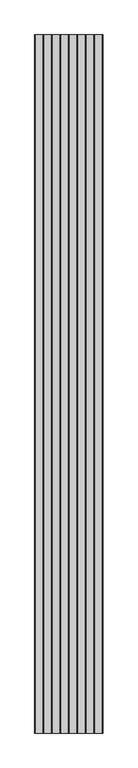
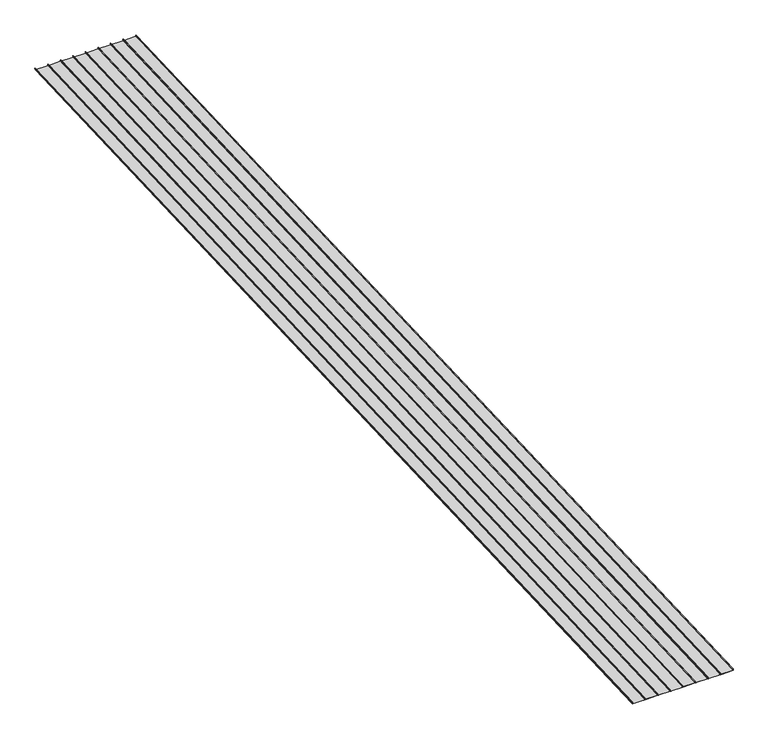
"""IFC4 building model written with IfcOpenShell, lengths in millimetres: proxy geometry, Generic Models 2:Generic Models 2:310765:Generic Models 2:310765 : Generic Models 2:Generic Models 2:310765:8 : Generic Models 2:Generic Models 2:310765:Generic Models 2:310765 : Generic Models 2:Generic Models 2:310765:300385."""

import ifcopenshell
import ifcopenshell.guid

model = None  # the IFC model being written
_history = None  # IfcOwnerHistory: only IFC2X3 demands one
_inside = {}  # id of a spatial element -> (the spatial element, [elements in it])
_under = {}  # id of a project, library or spatial element -> (it, [spatial elements below it])
_declared = {}  # id of a project -> (the project, [libraries it declares])
_typed = {}  # id of a type object -> (the type object, [elements of that type])
_made_of = {}  # id of a material, layer set ... -> (it, [elements and type objects made of it])


def new_model(schema):
    """Start an empty IFC model of exactly this schema.

    Asked for "IFC4X3", IfcOpenShell would pick the latest addendum, in which some entities
    have other attributes; the version numbers below select the first issue.
    IFC2X3 requires an IfcOwnerHistory on every rooted entity: one is made here for all.
    """
    global model, _history
    if schema == "IFC4X3":
        model = ifcopenshell.file(schema_version=(4, 3, 0, 0))
    else:
        model = ifcopenshell.file(schema=schema)
    _inside.clear()
    _under.clear()
    _declared.clear()
    _typed.clear()
    _made_of.clear()
    _history = None
    if model.schema == "IFC2X3":
        org = make("IfcOrganization", Name="unknown")
        user = make(
            "IfcPersonAndOrganization",
            ThePerson=make("IfcPerson", FamilyName="unknown"),
            TheOrganization=org,
        )
        app = make(
            "IfcApplication",
            ApplicationDeveloper=org,
            Version="unknown",
            ApplicationFullName="unknown",
            ApplicationIdentifier="unknown",
        )
        _history = make(
            "IfcOwnerHistory",
            OwningUser=user,
            OwningApplication=app,
            ChangeAction="ADDED",
            CreationDate=0,
        )
    return model


def make(cls, **values):
    """One entity of the class cls with the attributes given. An attribute that is None is left unset."""
    return model.create_entity(
        cls, **{name: value for name, value in values.items() if value is not None}
    )


def rooted(cls, **values):
    """An entity with a GlobalId (a new one), such as an element, a storey or a relation."""
    return make(cls, GlobalId=ifcopenshell.guid.new(), OwnerHistory=_history, **values)


def si_unit(unit_type, name, prefix=None):
    """IfcSIUnit, for example si_unit("LENGTHUNIT", "METRE", prefix="MILLI")."""
    return make("IfcSIUnit", UnitType=unit_type, Prefix=prefix, Name=name)


def assignment(units):
    """IfcUnitAssignment: the units of a project."""
    return None if units is None else make("IfcUnitAssignment", Units=units)


def point(xyz):
    """IfcCartesianPoint."""
    return None if xyz is None else make("IfcCartesianPoint", Coordinates=xyz)


def direction(xyz):
    """IfcDirection."""
    return None if xyz is None else make("IfcDirection", DirectionRatios=xyz)


def frame(location, z_axis=None, x_axis=None):
    """IfcAxis2Placement3D, a coordinate frame: its origin and axes. An axis left out is left unset."""
    return make(
        "IfcAxis2Placement3D",
        Location=point(location),
        Axis=direction(z_axis),
        RefDirection=direction(x_axis),
    )


def origin():
    """The frame at (0, 0, 0) with its axes left unset."""
    return frame((0.0, 0.0, 0.0))


def place(relative_to, where):
    """IfcLocalPlacement: puts the frame where relative to a parent placement (None: the world)."""
    return make(
        "IfcLocalPlacement", PlacementRelTo=relative_to, RelativePlacement=where
    )


def context(
    kind, dimensions, precision=None, world=None, true_north=None, identifier=None
):
    """IfcGeometricRepresentationContext, for example the 3D "Model" context."""
    return make(
        "IfcGeometricRepresentationContext",
        ContextIdentifier=identifier,
        ContextType=kind,
        CoordinateSpaceDimension=dimensions,
        Precision=precision,
        WorldCoordinateSystem=world,
        TrueNorth=true_north,
    )


def project(units=None, contexts=None):
    """IfcProject with its units and contexts."""
    return rooted(
        "IfcProject",
        Name="project",
        RepresentationContexts=contexts,
        UnitsInContext=assignment(units),
    )


def spatial(cls, under=None, at=None, **own):
    """A site, building, storey or space (cls), placed at a placement, below another one or the project."""
    s = rooted(cls, ObjectPlacement=at, **own)
    if under is not None:
        _under.setdefault(under.id(), (under, []))[1].append(s)
    return s


def polyline(points):
    """IfcPolyline through the points."""
    return make("IfcPolyline", Points=[point(p) for p in points])


def outline(outer, holes=None, kind="AREA"):
    """IfcArbitraryClosedProfileDef: a profile drawn as a closed curve; with holes, ...WithVoids."""
    if holes is None:
        return make("IfcArbitraryClosedProfileDef", ProfileType=kind, OuterCurve=outer)
    return make(
        "IfcArbitraryProfileDefWithVoids",
        ProfileType=kind,
        OuterCurve=outer,
        InnerCurves=holes,
    )


def extrude(swept, where, along, depth):
    """IfcExtrudedAreaSolid: the profile swept, set in the frame where, extruded along a direction by depth."""
    return make(
        "IfcExtrudedAreaSolid",
        SweptArea=swept,
        Position=where,
        ExtrudedDirection=direction(along),
        Depth=depth,
    )


def shape(context_of_items, identifier, shape_type, items):
    """IfcShapeRepresentation: the items that make up one representation, for example the "Body"."""
    return make(
        "IfcShapeRepresentation",
        ContextOfItems=context_of_items,
        RepresentationIdentifier=identifier,
        RepresentationType=shape_type,
        Items=items,
    )


def source(mapping_origin, context_of_items, identifier, shape_type, items):
    """IfcRepresentationMap: a shape defined once, which mapped items show again and again."""
    return make(
        "IfcRepresentationMap",
        MappingOrigin=mapping_origin,
        MappedRepresentation=shape(context_of_items, identifier, shape_type, items),
    )


def transform(
    local_origin,
    x_axis=None,
    y_axis=None,
    z_axis=None,
    scale=None,
    scale2=None,
    scale3=None,
    uniform=True,
):
    """IfcCartesianTransformationOperator3D, or its non-uniform kind. x_axis, y_axis, z_axis: its Axis1, 2, 3."""
    if uniform:
        return make(
            "IfcCartesianTransformationOperator3D",
            Axis1=direction(x_axis),
            Axis2=direction(y_axis),
            LocalOrigin=point(local_origin),
            Scale=scale,
            Axis3=direction(z_axis),
        )
    return make(
        "IfcCartesianTransformationOperator3DnonUniform",
        Axis1=direction(x_axis),
        Axis2=direction(y_axis),
        LocalOrigin=point(local_origin),
        Scale=scale,
        Axis3=direction(z_axis),
        Scale2=scale2,
        Scale3=scale3,
    )


def mapped(mapping_source, mapping_target):
    """IfcMappedItem: shows the shape of a source again, moved by a transform."""
    return make(
        "IfcMappedItem", MappingSource=mapping_source, MappingTarget=mapping_target
    )


def made_of(thing, what):
    """Note that an element or type object is made of a material, layer set ...; save() writes the relation."""
    if what is not None:
        _made_of.setdefault(what.id(), (what, []))[1].append(thing)
    return thing


def element(
    cls,
    number,
    at=None,
    inside=None,
    cuts=None,
    type_object=None,
    material=None,
    context=None,
    identifier="Body",
    shape_type=None,
    held_by="IfcProductDefinitionShape",
    body=None,
    shapes=None,
    **own,
):
    """One element of the class cls, such as IfcWall. Its Tag is "e" and its number.

    at: its placement. inside: the storey or other place that contains it. cuts: it is an
    opening in that element (IfcRelVoidsElement). A single representation is given by context,
    identifier, shape_type and body (its items); several are given by shapes. held_by: the class
    of the entity that holds the representations. save() writes the other relations.
    """
    e = rooted(cls, Tag="e%d" % number, ObjectPlacement=at, **own)
    if body is not None:
        shapes = [shape(context, identifier, shape_type, body)]
    if shapes is not None:
        e.Representation = make(held_by, Representations=shapes)
    if inside is not None:
        _inside.setdefault(inside.id(), (inside, []))[1].append(e)
    if cuts is not None:
        rooted(
            "IfcRelVoidsElement", RelatingBuildingElement=cuts, RelatedOpeningElement=e
        )
    if type_object is not None:
        _typed.setdefault(type_object.id(), (type_object, []))[1].append(e)
    return made_of(e, material)


def aggregate(whole, parts):
    """IfcRelAggregates: a whole, such as a stair, and the parts it consists of."""
    return rooted("IfcRelAggregates", RelatingObject=whole, RelatedObjects=parts)


def save(model, path):
    """Write the relations noted so far, then the file.

    IfcRelAggregates (storeys below a building ...), IfcRelContainedInSpatialStructure (elements
    in a storey), IfcRelDefinesByType, IfcRelAssociatesMaterial and IfcRelDeclares: one each for
    every whole, place, type object, material and project.
    """
    for whole, parts in _under.values():
        aggregate(whole, parts)
    for where, things in _inside.values():
        rooted(
            "IfcRelContainedInSpatialStructure",
            RelatedElements=things,
            RelatingStructure=where,
        )
    for kind, things in _typed.values():
        rooted("IfcRelDefinesByType", RelatedObjects=things, RelatingType=kind)
    for what, things in _made_of.values():
        rooted("IfcRelAssociatesMaterial", RelatedObjects=things, RelatingMaterial=what)
    for by, libraries in _declared.values():
        rooted("IfcRelDeclares", RelatingContext=by, RelatedDefinitions=libraries)
    model.write(path)


def generic_models_05e155ed(model_context):
    return source(origin(), model_context, "Body", "SweptSolid", [
        extrude(outline(polyline([(1.5875, 0.0), (1.5875, 50.8), (406.4, 50.8), (406.4, 1.5874999), (395.2875, 1.5874999), (395.2875, 11.1124999), (396.875, 11.1124999), (396.875, 3.175), (404.8125, 3.175), (404.8125, 49.2124999), (3.175, 49.2124999), (3.175, -1.5875), (-14.2875, -1.5875), (-14.2875, 9.525), (-12.7, 9.525), (-12.7, 0.0), (1.5875, 0.0)])), frame((594966.8117242, -569895.5205486, 8783.336734), z_axis=(0.0, 0.9991330730923568, 0.04163054471206784), x_axis=(1.0, 0.0, 0.0)), (0.0, 0.0, 1.0), 33445.8614342),
        extrude(outline(polyline([(-404.8125, 0.0), (-404.8125, 50.8), (0.0, 50.8), (0.0, 1.5874999), (-11.1125, 1.5874999), (-11.1125, 11.1124999), (-9.525, 11.1124999), (-9.525, 3.175), (-1.5875, 3.175), (-1.5875, 49.2124999), (-403.225, 49.2124999), (-403.225, -1.5875), (-420.6875, -1.5875), (-420.6875, 9.525), (-419.1, 9.525), (-419.1, 0.0), (-404.8125, 0.0)])), frame((594966.8117242, -569895.5205486, 8783.336734), z_axis=(0.0, 0.9991330730923568, 0.04163054471206784), x_axis=(1.0, 0.0, 0.0)), (0.0, 0.0, 1.0), 33445.8614342),
        extrude(outline(polyline([(-811.2125, 0.0), (-811.2125, 50.8), (-406.4, 50.8), (-406.4, 1.5874999), (-417.5125, 1.5874999), (-417.5125, 11.1124999), (-415.925, 11.1124999), (-415.925, 3.175), (-407.9875, 3.175), (-407.9875, 49.2124999), (-809.625, 49.2124999), (-809.625, -1.5875), (-827.0875, -1.5875), (-827.0875, 9.525), (-825.5, 9.525), (-825.5, 0.0), (-811.2125, 0.0)])), frame((594966.8117242, -569895.5205486, 8783.336734), z_axis=(0.0, 0.9991330730923568, 0.04163054471206784), x_axis=(1.0, 0.0, 0.0)), (0.0, 0.0, 1.0), 33445.8614342),
        extrude(outline(polyline([(-1217.6125, 0.0), (-1217.6125, 50.8), (-812.8, 50.8), (-812.8, 1.5874999), (-823.9125, 1.5874999), (-823.9125, 11.1124999), (-822.325, 11.1124999), (-822.325, 3.175), (-814.3875, 3.175), (-814.3875, 49.2124999), (-1216.025, 49.2124999), (-1216.025, -1.5875), (-1233.4875, -1.5875), (-1233.4875, 9.525), (-1231.9, 9.525), (-1231.9, 0.0), (-1217.6125, 0.0)])), frame((594966.8117242, -569895.5205486, 8783.336734), z_axis=(0.0, 0.9991330730923568, 0.04163054471206784), x_axis=(1.0, 0.0, 0.0)), (0.0, 0.0, 1.0), 33445.8614342),
        extrude(outline(polyline([(-1624.0125, 0.0), (-1624.0125, 50.8), (-1219.2, 50.8), (-1219.2, 1.5874999), (-1230.3125, 1.5874999), (-1230.3125, 11.1124999), (-1228.725, 11.1124999), (-1228.725, 3.175), (-1220.7875, 3.175), (-1220.7875, 49.2124999), (-1622.425, 49.2124999), (-1622.425, -1.5875), (-1639.8875, -1.5875), (-1639.8875, 9.525), (-1638.3, 9.525), (-1638.3, 0.0), (-1624.0125, 0.0)])), frame((594966.8117242, -569895.5205486, 8783.336734), z_axis=(0.0, 0.9991330730923568, 0.04163054471206784), x_axis=(1.0, 0.0, 0.0)), (0.0, 0.0, 1.0), 33445.8614342),
        extrude(outline(polyline([(-2030.4125, 0.0), (-2030.4125, 50.8), (-1625.6, 50.8), (-1625.6, 1.5874999), (-1636.7125, 1.5874999), (-1636.7125, 11.1124999), (-1635.125, 11.1124999), (-1635.125, 3.175), (-1627.1875, 3.175), (-1627.1875, 49.2124999), (-2028.825, 49.2124999), (-2028.825, -1.5875), (-2046.2875, -1.5875), (-2046.2875, 9.525), (-2044.7, 9.525), (-2044.7, 0.0), (-2030.4125, 0.0)])), frame((594966.8117242, -569895.5205486, 8783.336734), z_axis=(0.0, 0.9991330730923568, 0.04163054471206784), x_axis=(1.0, 0.0, 0.0)), (0.0, 0.0, 1.0), 33445.8614342),
        extrude(outline(polyline([(-2436.8125, 0.0), (-2436.8125, 50.8), (-2032.0, 50.8), (-2032.0, 1.5874999), (-2043.1125, 1.5874999), (-2043.1125, 11.1124999), (-2041.525, 11.1124999), (-2041.525, 3.175), (-2033.5875, 3.175), (-2033.5875, 49.2124999), (-2435.225, 49.2124999), (-2435.225, -1.5875), (-2452.6875, -1.5875), (-2452.6875, 9.525), (-2451.1, 9.525), (-2451.1, 0.0), (-2436.8125, 0.0)])), frame((594966.8117242, -569895.5205486, 8783.336734), z_axis=(0.0, 0.9991330730923568, 0.04163054471206784), x_axis=(1.0, 0.0, 0.0)), (0.0, 0.0, 1.0), 33445.8614342),
        extrude(outline(polyline([(-2843.2125, 0.0), (-2843.2125, 50.8), (-2438.4, 50.8), (-2438.4, 1.5874999), (-2449.5125, 1.5874999), (-2449.5125, 11.1124999), (-2447.925, 11.1124999), (-2447.925, 3.175), (-2439.9875, 3.175), (-2439.9875, 49.2124999), (-2841.625, 49.2124999), (-2841.625, -1.5875), (-2859.0875, -1.5875), (-2859.0875, 9.525), (-2857.5, 9.525), (-2857.5, 0.0), (-2843.2125, 0.0)])), frame((594966.8117242, -569895.5205486, 8783.336734), z_axis=(0.0, 0.9991330730923568, 0.04163054471206784), x_axis=(1.0, 0.0, 0.0)), (0.0, 0.0, 1.0), 33445.8614342),
    ])


if __name__ == "__main__":
    model = new_model("IFC4")
    model_context = context("Model", 3, world=origin())
    ifc_project = project(units=[si_unit("LENGTHUNIT", "METRE", prefix="MILLI")], contexts=[model_context])
    site = spatial("IfcSite", under=ifc_project)
    building = spatial("IfcBuilding", under=site)
    placement = place(None, origin())
    generic_models_shape = generic_models_05e155ed(model_context)
    element("IfcBuildingElementProxy", 1, Name="Generic Models 2:Generic Models 2:310765:Generic Models 2:310765 : Generic Models 2:Generic Models 2:310765:8 : Generic Models 2:Generic Models 2:310765:Generic Models 2:310765 : Generic Models 2:Generic Models 2:310765:300385", ObjectType="Generic Models 2:Generic Models 2:310765:Generic Models 2:310765 : Generic Models 2:Generic Models 2:310765:8 : Generic Models 2:Generic Models 2:310765:Generic Models 2:310765 : Generic Models 2:Generic Models 2:310765:300385", at=placement, inside=building, context=model_context, shape_type="MappedRepresentation", body=[
        mapped(generic_models_shape, transform((0.0, 0.0, 0.0), x_axis=(1.0, 0.0, 0.0), y_axis=(0.0, 1.0, 0.0), z_axis=(0.0, 0.0, 1.0))),
    ])
    save(model, "model.ifc")

# Revit data of these elements
# Type "Generic Models 2:Generic Models 2:310765:Generic Models 2:310765 : Generic Models 2:Generic Models 2:310765:8 : Generic Models 2:Generic Models 2:310765:Generic Models 2:310765 : Generic Models 2:Generic Models 2:310765:300385"
#   NameOverride = "Generic Models 2:Generic Models 2:310765:Generic Models 2:310765 : Generic Models 2:Generic Models 2:310765:300385"
#   ObjectTypeOverride = "Generic Models 2:310765 : Generic Models 2:Generic Models 2:310765"
#   Reference = "Generic Models 2"
#   Tag = "300385"
# Element 1 (IfcBuildingElementProxy, "Generic Models 2:Generic Models 2:310765:Generic Models 2:310765 : Generic Models 2:Generic Models 2:310765:8 : Generic Models 2:Generic Models 2:310765:Generic Models 2:310765 : Generic Models 2:Generic Models 2:310765:300385")
#   Materials on its faces: "STRUCTURAL STANDING SEAM SHEET METAL ROOFING - DOUBLE-LOK - COLOR T.B.D."
# Materials
#   "STRUCTURAL STANDING SEAM SHEET METAL ROOFING - DOUBLE-LOK - COLOR T.B.D.": class "Generic", colour RGB 120 120 120, transparency 0, Cost = 0
